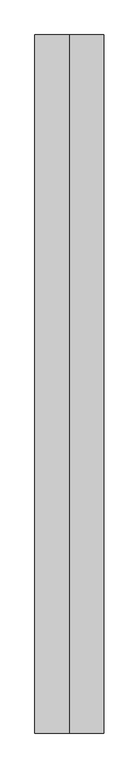
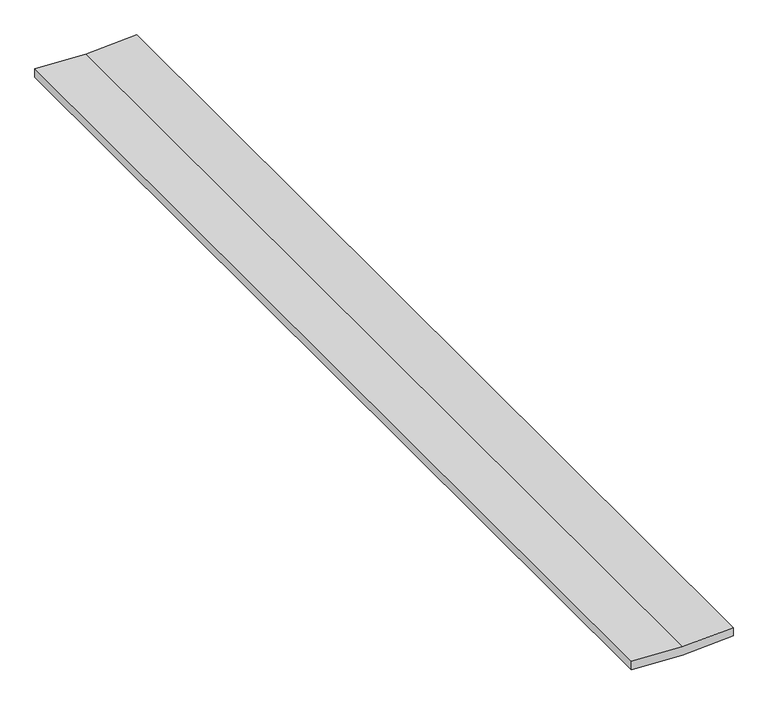
"""IFC4 building model written with IfcOpenShell, lengths in millimetres: proxy geometry, COVER BOARD001 3887 : COVER BOARD001 3887."""

import ifcopenshell
import ifcopenshell.guid

model = None  # the IFC model being written
_history = None  # IfcOwnerHistory: only IFC2X3 demands one
_inside = {}  # id of a spatial element -> (the spatial element, [elements in it])
_under = {}  # id of a project, library or spatial element -> (it, [spatial elements below it])
_declared = {}  # id of a project -> (the project, [libraries it declares])
_typed = {}  # id of a type object -> (the type object, [elements of that type])
_made_of = {}  # id of a material, layer set ... -> (it, [elements and type objects made of it])


def new_model(schema):
    """Start an empty IFC model of exactly this schema.

    Asked for "IFC4X3", IfcOpenShell would pick the latest addendum, in which some entities
    have other attributes; the version numbers below select the first issue.
    IFC2X3 requires an IfcOwnerHistory on every rooted entity: one is made here for all.
    """
    global model, _history
    if schema == "IFC4X3":
        model = ifcopenshell.file(schema_version=(4, 3, 0, 0))
    else:
        model = ifcopenshell.file(schema=schema)
    _inside.clear()
    _under.clear()
    _declared.clear()
    _typed.clear()
    _made_of.clear()
    _history = None
    if model.schema == "IFC2X3":
        org = make("IfcOrganization", Name="unknown")
        user = make(
            "IfcPersonAndOrganization",
            ThePerson=make("IfcPerson", FamilyName="unknown"),
            TheOrganization=org,
        )
        app = make(
            "IfcApplication",
            ApplicationDeveloper=org,
            Version="unknown",
            ApplicationFullName="unknown",
            ApplicationIdentifier="unknown",
        )
        _history = make(
            "IfcOwnerHistory",
            OwningUser=user,
            OwningApplication=app,
            ChangeAction="ADDED",
            CreationDate=0,
        )
    return model


def make(cls, **values):
    """One entity of the class cls with the attributes given. An attribute that is None is left unset."""
    return model.create_entity(
        cls, **{name: value for name, value in values.items() if value is not None}
    )


def rooted(cls, **values):
    """An entity with a GlobalId (a new one), such as an element, a storey or a relation."""
    return make(cls, GlobalId=ifcopenshell.guid.new(), OwnerHistory=_history, **values)


def si_unit(unit_type, name, prefix=None):
    """IfcSIUnit, for example si_unit("LENGTHUNIT", "METRE", prefix="MILLI")."""
    return make("IfcSIUnit", UnitType=unit_type, Prefix=prefix, Name=name)


def assignment(units):
    """IfcUnitAssignment: the units of a project."""
    return None if units is None else make("IfcUnitAssignment", Units=units)


def point(xyz):
    """IfcCartesianPoint."""
    return None if xyz is None else make("IfcCartesianPoint", Coordinates=xyz)


def direction(xyz):
    """IfcDirection."""
    return None if xyz is None else make("IfcDirection", DirectionRatios=xyz)


def frame(location, z_axis=None, x_axis=None):
    """IfcAxis2Placement3D, a coordinate frame: its origin and axes. An axis left out is left unset."""
    return make(
        "IfcAxis2Placement3D",
        Location=point(location),
        Axis=direction(z_axis),
        RefDirection=direction(x_axis),
    )


def origin():
    """The frame at (0, 0, 0) with its axes left unset."""
    return frame((0.0, 0.0, 0.0))


def place(relative_to, where):
    """IfcLocalPlacement: puts the frame where relative to a parent placement (None: the world)."""
    return make(
        "IfcLocalPlacement", PlacementRelTo=relative_to, RelativePlacement=where
    )


def context(
    kind, dimensions, precision=None, world=None, true_north=None, identifier=None
):
    """IfcGeometricRepresentationContext, for example the 3D "Model" context."""
    return make(
        "IfcGeometricRepresentationContext",
        ContextIdentifier=identifier,
        ContextType=kind,
        CoordinateSpaceDimension=dimensions,
        Precision=precision,
        WorldCoordinateSystem=world,
        TrueNorth=true_north,
    )


def project(units=None, contexts=None):
    """IfcProject with its units and contexts."""
    return rooted(
        "IfcProject",
        Name="project",
        RepresentationContexts=contexts,
        UnitsInContext=assignment(units),
    )


def spatial(cls, under=None, at=None, **own):
    """A site, building, storey or space (cls), placed at a placement, below another one or the project."""
    s = rooted(cls, ObjectPlacement=at, **own)
    if under is not None:
        _under.setdefault(under.id(), (under, []))[1].append(s)
    return s


def polyline(points):
    """IfcPolyline through the points."""
    return make("IfcPolyline", Points=[point(p) for p in points])


def outline(outer, holes=None, kind="AREA"):
    """IfcArbitraryClosedProfileDef: a profile drawn as a closed curve; with holes, ...WithVoids."""
    if holes is None:
        return make("IfcArbitraryClosedProfileDef", ProfileType=kind, OuterCurve=outer)
    return make(
        "IfcArbitraryProfileDefWithVoids",
        ProfileType=kind,
        OuterCurve=outer,
        InnerCurves=holes,
    )


def extrude(swept, where, along, depth):
    """IfcExtrudedAreaSolid: the profile swept, set in the frame where, extruded along a direction by depth."""
    return make(
        "IfcExtrudedAreaSolid",
        SweptArea=swept,
        Position=where,
        ExtrudedDirection=direction(along),
        Depth=depth,
    )


def shape(context_of_items, identifier, shape_type, items):
    """IfcShapeRepresentation: the items that make up one representation, for example the "Body"."""
    return make(
        "IfcShapeRepresentation",
        ContextOfItems=context_of_items,
        RepresentationIdentifier=identifier,
        RepresentationType=shape_type,
        Items=items,
    )


def source(mapping_origin, context_of_items, identifier, shape_type, items):
    """IfcRepresentationMap: a shape defined once, which mapped items show again and again."""
    return make(
        "IfcRepresentationMap",
        MappingOrigin=mapping_origin,
        MappedRepresentation=shape(context_of_items, identifier, shape_type, items),
    )


def transform(
    local_origin,
    x_axis=None,
    y_axis=None,
    z_axis=None,
    scale=None,
    scale2=None,
    scale3=None,
    uniform=True,
):
    """IfcCartesianTransformationOperator3D, or its non-uniform kind. x_axis, y_axis, z_axis: its Axis1, 2, 3."""
    if uniform:
        return make(
            "IfcCartesianTransformationOperator3D",
            Axis1=direction(x_axis),
            Axis2=direction(y_axis),
            LocalOrigin=point(local_origin),
            Scale=scale,
            Axis3=direction(z_axis),
        )
    return make(
        "IfcCartesianTransformationOperator3DnonUniform",
        Axis1=direction(x_axis),
        Axis2=direction(y_axis),
        LocalOrigin=point(local_origin),
        Scale=scale,
        Axis3=direction(z_axis),
        Scale2=scale2,
        Scale3=scale3,
    )


def mapped(mapping_source, mapping_target):
    """IfcMappedItem: shows the shape of a source again, moved by a transform."""
    return make(
        "IfcMappedItem", MappingSource=mapping_source, MappingTarget=mapping_target
    )


def made_of(thing, what):
    """Note that an element or type object is made of a material, layer set ...; save() writes the relation."""
    if what is not None:
        _made_of.setdefault(what.id(), (what, []))[1].append(thing)
    return thing


def element(
    cls,
    number,
    at=None,
    inside=None,
    cuts=None,
    type_object=None,
    material=None,
    context=None,
    identifier="Body",
    shape_type=None,
    held_by="IfcProductDefinitionShape",
    body=None,
    shapes=None,
    **own,
):
    """One element of the class cls, such as IfcWall. Its Tag is "e" and its number.

    at: its placement. inside: the storey or other place that contains it. cuts: it is an
    opening in that element (IfcRelVoidsElement). A single representation is given by context,
    identifier, shape_type and body (its items); several are given by shapes. held_by: the class
    of the entity that holds the representations. save() writes the other relations.
    """
    e = rooted(cls, Tag="e%d" % number, ObjectPlacement=at, **own)
    if body is not None:
        shapes = [shape(context, identifier, shape_type, body)]
    if shapes is not None:
        e.Representation = make(held_by, Representations=shapes)
    if inside is not None:
        _inside.setdefault(inside.id(), (inside, []))[1].append(e)
    if cuts is not None:
        rooted(
            "IfcRelVoidsElement", RelatingBuildingElement=cuts, RelatedOpeningElement=e
        )
    if type_object is not None:
        _typed.setdefault(type_object.id(), (type_object, []))[1].append(e)
    return made_of(e, material)


def aggregate(whole, parts):
    """IfcRelAggregates: a whole, such as a stair, and the parts it consists of."""
    return rooted("IfcRelAggregates", RelatingObject=whole, RelatedObjects=parts)


def save(model, path):
    """Write the relations noted so far, then the file.

    IfcRelAggregates (storeys below a building ...), IfcRelContainedInSpatialStructure (elements
    in a storey), IfcRelDefinesByType, IfcRelAssociatesMaterial and IfcRelDeclares: one each for
    every whole, place, type object, material and project.
    """
    for whole, parts in _under.values():
        aggregate(whole, parts)
    for where, things in _inside.values():
        rooted(
            "IfcRelContainedInSpatialStructure",
            RelatedElements=things,
            RelatingStructure=where,
        )
    for kind, things in _typed.values():
        rooted("IfcRelDefinesByType", RelatedObjects=things, RelatingType=kind)
    for what, things in _made_of.values():
        rooted("IfcRelAssociatesMaterial", RelatedObjects=things, RelatingMaterial=what)
    for by, libraries in _declared.values():
        rooted("IfcRelDeclares", RelatingContext=by, RelatedDefinitions=libraries)
    model.write(path)


def generic_models_2390c736(model_context):
    return source(origin(), model_context, "Body", "SweptSolid", [
        extrude(outline(polyline([(40228.3444286, -4699.8063764), (40233.346, -4797.9038825), (40216.0142809, -4797.9038825), (40211.0127094, -4699.8063764), (40216.0142809, -4601.0538825), (40233.346, -4601.0538825), (40228.3444286, -4699.8063764)])), frame((0.0, -1052.6406573, 0.0), z_axis=(0.0, 1.0, 0.0), x_axis=(0.0, 0.0, 1.0)), (0.0, 0.0, 1.0), 2000.0),
    ])


if __name__ == "__main__":
    model = new_model("IFC4")
    model_context = context("Model", 3, world=origin())
    ifc_project = project(units=[si_unit("LENGTHUNIT", "METRE", prefix="MILLI")], contexts=[model_context])
    site = spatial("IfcSite", under=ifc_project)
    building = spatial("IfcBuilding", under=site)
    placement = place(None, origin())
    generic_models_shape = generic_models_2390c736(model_context)
    element("IfcBuildingElementProxy", 1, Name="COVER BOARD001 3887 : COVER BOARD001 3887", ObjectType="COVER BOARD001 3887 : COVER BOARD001 3887", at=placement, inside=building, context=model_context, shape_type="MappedRepresentation", body=[
        mapped(generic_models_shape, transform((0.0, 0.0, 0.0), x_axis=(1.0, 0.0, 0.0), y_axis=(0.0, 1.0, 0.0), z_axis=(0.0, 0.0, 1.0))),
    ])
    save(model, "model.ifc")

# Revit data of these elements
# Type "COVER BOARD001 3887 : COVER BOARD001 3887"
#   NameOverride = "COVER BOARD001"
# Element 1 (IfcBuildingElementProxy, "COVER BOARD001 3887 : COVER BOARD001 3887")
#   Materials on its faces: "CDX PLYWOOD - SEE STRUCTURAL DWGS"
# Materials
#   "CDX PLYWOOD - SEE STRUCTURAL DWGS": class "Unassigned", colour RGB 138 93 50, transparency 0, Cost = 0
